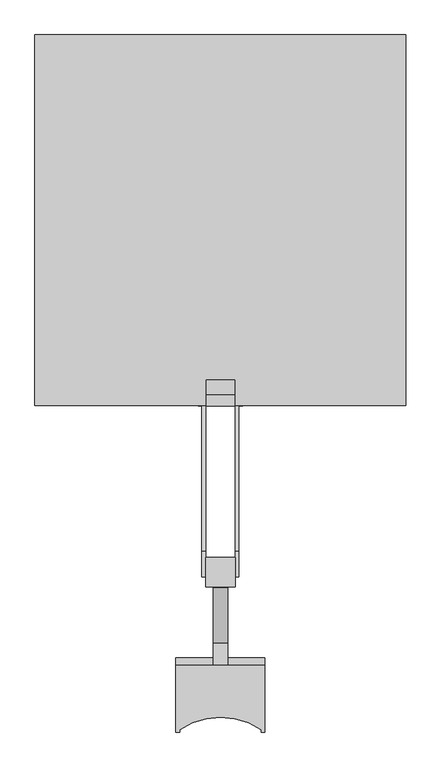
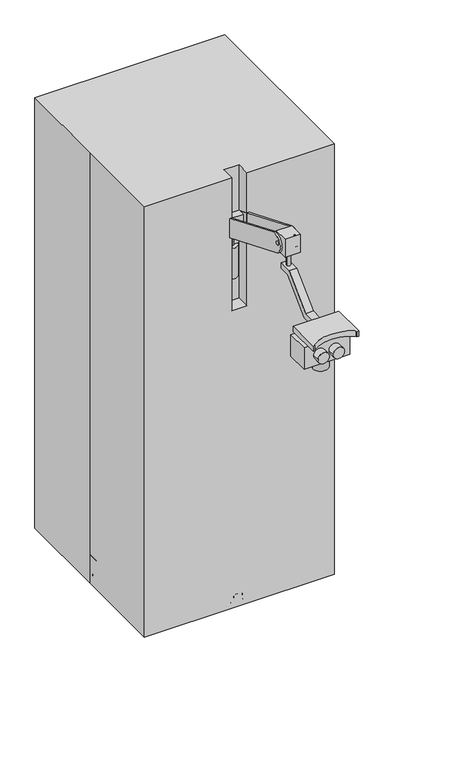
"""IFC4 building model written with IfcOpenShell, lengths in millimetres: proxy geometry, M8535 - Microscope, Operating, Portable : M8535 - Microscope, Operating, Portable."""

import ifcopenshell
import ifcopenshell.guid

model = None  # the IFC model being written
_history = None  # IfcOwnerHistory: only IFC2X3 demands one
_inside = {}  # id of a spatial element -> (the spatial element, [elements in it])
_under = {}  # id of a project, library or spatial element -> (it, [spatial elements below it])
_declared = {}  # id of a project -> (the project, [libraries it declares])
_typed = {}  # id of a type object -> (the type object, [elements of that type])
_made_of = {}  # id of a material, layer set ... -> (it, [elements and type objects made of it])


def new_model(schema):
    """Start an empty IFC model of exactly this schema.

    Asked for "IFC4X3", IfcOpenShell would pick the latest addendum, in which some entities
    have other attributes; the version numbers below select the first issue.
    IFC2X3 requires an IfcOwnerHistory on every rooted entity: one is made here for all.
    """
    global model, _history
    if schema == "IFC4X3":
        model = ifcopenshell.file(schema_version=(4, 3, 0, 0))
    else:
        model = ifcopenshell.file(schema=schema)
    _inside.clear()
    _under.clear()
    _declared.clear()
    _typed.clear()
    _made_of.clear()
    _history = None
    if model.schema == "IFC2X3":
        org = make("IfcOrganization", Name="unknown")
        user = make(
            "IfcPersonAndOrganization",
            ThePerson=make("IfcPerson", FamilyName="unknown"),
            TheOrganization=org,
        )
        app = make(
            "IfcApplication",
            ApplicationDeveloper=org,
            Version="unknown",
            ApplicationFullName="unknown",
            ApplicationIdentifier="unknown",
        )
        _history = make(
            "IfcOwnerHistory",
            OwningUser=user,
            OwningApplication=app,
            ChangeAction="ADDED",
            CreationDate=0,
        )
    return model


def make(cls, **values):
    """One entity of the class cls with the attributes given. An attribute that is None is left unset."""
    return model.create_entity(
        cls, **{name: value for name, value in values.items() if value is not None}
    )


def rooted(cls, **values):
    """An entity with a GlobalId (a new one), such as an element, a storey or a relation."""
    return make(cls, GlobalId=ifcopenshell.guid.new(), OwnerHistory=_history, **values)


def si_unit(unit_type, name, prefix=None):
    """IfcSIUnit, for example si_unit("LENGTHUNIT", "METRE", prefix="MILLI")."""
    return make("IfcSIUnit", UnitType=unit_type, Prefix=prefix, Name=name)


def assignment(units):
    """IfcUnitAssignment: the units of a project."""
    return None if units is None else make("IfcUnitAssignment", Units=units)


def point(xyz):
    """IfcCartesianPoint."""
    return None if xyz is None else make("IfcCartesianPoint", Coordinates=xyz)


def direction(xyz):
    """IfcDirection."""
    return None if xyz is None else make("IfcDirection", DirectionRatios=xyz)


def frame(location, z_axis=None, x_axis=None):
    """IfcAxis2Placement3D, a coordinate frame: its origin and axes. An axis left out is left unset."""
    return make(
        "IfcAxis2Placement3D",
        Location=point(location),
        Axis=direction(z_axis),
        RefDirection=direction(x_axis),
    )


def frame_2d(location, x_axis=None):
    """IfcAxis2Placement2D, a coordinate frame in the plane: its origin and x axis."""
    return make(
        "IfcAxis2Placement2D", Location=point(location), RefDirection=direction(x_axis)
    )


def origin():
    """The frame at (0, 0, 0) with its axes left unset."""
    return frame((0.0, 0.0, 0.0))


def origin_2d():
    """The frame at (0, 0) in the plane with its x axis left unset."""
    return frame_2d((0.0, 0.0))


def place(relative_to, where):
    """IfcLocalPlacement: puts the frame where relative to a parent placement (None: the world)."""
    return make(
        "IfcLocalPlacement", PlacementRelTo=relative_to, RelativePlacement=where
    )


def context(
    kind, dimensions, precision=None, world=None, true_north=None, identifier=None
):
    """IfcGeometricRepresentationContext, for example the 3D "Model" context."""
    return make(
        "IfcGeometricRepresentationContext",
        ContextIdentifier=identifier,
        ContextType=kind,
        CoordinateSpaceDimension=dimensions,
        Precision=precision,
        WorldCoordinateSystem=world,
        TrueNorth=true_north,
    )


def project(units=None, contexts=None):
    """IfcProject with its units and contexts."""
    return rooted(
        "IfcProject",
        Name="project",
        RepresentationContexts=contexts,
        UnitsInContext=assignment(units),
    )


def spatial(cls, under=None, at=None, **own):
    """A site, building, storey or space (cls), placed at a placement, below another one or the project."""
    s = rooted(cls, ObjectPlacement=at, **own)
    if under is not None:
        _under.setdefault(under.id(), (under, []))[1].append(s)
    return s


def polyline(points):
    """IfcPolyline through the points."""
    return make("IfcPolyline", Points=[point(p) for p in points])


def circle_curve(where, radius):
    """IfcCircle in the frame where."""
    return make("IfcCircle", Position=where, Radius=radius)


def ellipse_curve(where, semi_axis1, semi_axis2):
    """IfcEllipse in the frame where."""
    return make(
        "IfcEllipse", Position=where, SemiAxis1=semi_axis1, SemiAxis2=semi_axis2
    )


def trimmed(basis, trim1, trim2, sense, master):
    """IfcTrimmedCurve: the piece of a basis curve between two trims."""
    return make(
        "IfcTrimmedCurve",
        BasisCurve=basis,
        Trim1=trim1,
        Trim2=trim2,
        SenseAgreement=sense,
        MasterRepresentation=master,
    )


def segment(curve, same_sense, transition):
    """IfcCompositeCurveSegment."""
    return make(
        "IfcCompositeCurveSegment",
        Transition=transition,
        SameSense=same_sense,
        ParentCurve=curve,
    )


def composite_curve(segments, self_intersect=None):
    """IfcCompositeCurve: segments joined end to end."""
    return make("IfcCompositeCurve", Segments=segments, SelfIntersect=self_intersect)


def outline(outer, holes=None, kind="AREA"):
    """IfcArbitraryClosedProfileDef: a profile drawn as a closed curve; with holes, ...WithVoids."""
    if holes is None:
        return make("IfcArbitraryClosedProfileDef", ProfileType=kind, OuterCurve=outer)
    return make(
        "IfcArbitraryProfileDefWithVoids",
        ProfileType=kind,
        OuterCurve=outer,
        InnerCurves=holes,
    )


def extrude(swept, where, along, depth):
    """IfcExtrudedAreaSolid: the profile swept, set in the frame where, extruded along a direction by depth."""
    return make(
        "IfcExtrudedAreaSolid",
        SweptArea=swept,
        Position=where,
        ExtrudedDirection=direction(along),
        Depth=depth,
    )


def faces_of(points, faces, orient=None, outer=None):
    """IfcFace entities. A face is a list of loops; a loop is a list of indices into points, from 0.

    orient and outer hold one flag for each loop. By default every Orientation is true, the
    first loop of a face is its IfcFaceOuterBound and the others are IfcFaceBound.
    """
    made = []
    for i, loops in enumerate(faces):
        bounds = []
        for j, loop in enumerate(loops):
            is_outer = j == 0 if outer is None else outer[i][j]
            bounds.append(
                make(
                    "IfcFaceOuterBound" if is_outer else "IfcFaceBound",
                    Bound=make("IfcPolyLoop", Polygon=[points[k] for k in loop]),
                    Orientation=True if orient is None else orient[i][j],
                )
            )
        made.append(make("IfcFace", Bounds=bounds))
    return made


def faceted_brep(points, faces, orient=None, outer=None, voids=None):
    """IfcFacetedBrep: a solid bounded by flat faces; with voids (closed shells), ...WithVoids."""
    shared = [point(p) for p in points]
    hull = make("IfcClosedShell", CfsFaces=faces_of(shared, faces, orient, outer))
    if voids is None:
        return make("IfcFacetedBrep", Outer=hull)
    return make(
        "IfcFacetedBrepWithVoids",
        Outer=hull,
        Voids=[
            make(cls, CfsFaces=faces_of(shared, fs, o, b)) for cls, fs, o, b in voids
        ],
    )


def shape(context_of_items, identifier, shape_type, items):
    """IfcShapeRepresentation: the items that make up one representation, for example the "Body"."""
    return make(
        "IfcShapeRepresentation",
        ContextOfItems=context_of_items,
        RepresentationIdentifier=identifier,
        RepresentationType=shape_type,
        Items=items,
    )


def source(mapping_origin, context_of_items, identifier, shape_type, items):
    """IfcRepresentationMap: a shape defined once, which mapped items show again and again."""
    return make(
        "IfcRepresentationMap",
        MappingOrigin=mapping_origin,
        MappedRepresentation=shape(context_of_items, identifier, shape_type, items),
    )


def transform(
    local_origin,
    x_axis=None,
    y_axis=None,
    z_axis=None,
    scale=None,
    scale2=None,
    scale3=None,
    uniform=True,
):
    """IfcCartesianTransformationOperator3D, or its non-uniform kind. x_axis, y_axis, z_axis: its Axis1, 2, 3."""
    if uniform:
        return make(
            "IfcCartesianTransformationOperator3D",
            Axis1=direction(x_axis),
            Axis2=direction(y_axis),
            LocalOrigin=point(local_origin),
            Scale=scale,
            Axis3=direction(z_axis),
        )
    return make(
        "IfcCartesianTransformationOperator3DnonUniform",
        Axis1=direction(x_axis),
        Axis2=direction(y_axis),
        LocalOrigin=point(local_origin),
        Scale=scale,
        Axis3=direction(z_axis),
        Scale2=scale2,
        Scale3=scale3,
    )


def mapped(mapping_source, mapping_target):
    """IfcMappedItem: shows the shape of a source again, moved by a transform."""
    return make(
        "IfcMappedItem", MappingSource=mapping_source, MappingTarget=mapping_target
    )


def made_of(thing, what):
    """Note that an element or type object is made of a material, layer set ...; save() writes the relation."""
    if what is not None:
        _made_of.setdefault(what.id(), (what, []))[1].append(thing)
    return thing


def element(
    cls,
    number,
    at=None,
    inside=None,
    cuts=None,
    type_object=None,
    material=None,
    context=None,
    identifier="Body",
    shape_type=None,
    held_by="IfcProductDefinitionShape",
    body=None,
    shapes=None,
    **own,
):
    """One element of the class cls, such as IfcWall. Its Tag is "e" and its number.

    at: its placement. inside: the storey or other place that contains it. cuts: it is an
    opening in that element (IfcRelVoidsElement). A single representation is given by context,
    identifier, shape_type and body (its items); several are given by shapes. held_by: the class
    of the entity that holds the representations. save() writes the other relations.
    """
    e = rooted(cls, Tag="e%d" % number, ObjectPlacement=at, **own)
    if body is not None:
        shapes = [shape(context, identifier, shape_type, body)]
    if shapes is not None:
        e.Representation = make(held_by, Representations=shapes)
    if inside is not None:
        _inside.setdefault(inside.id(), (inside, []))[1].append(e)
    if cuts is not None:
        rooted(
            "IfcRelVoidsElement", RelatingBuildingElement=cuts, RelatedOpeningElement=e
        )
    if type_object is not None:
        _typed.setdefault(type_object.id(), (type_object, []))[1].append(e)
    return made_of(e, material)


def aggregate(whole, parts):
    """IfcRelAggregates: a whole, such as a stair, and the parts it consists of."""
    return rooted("IfcRelAggregates", RelatingObject=whole, RelatedObjects=parts)


def save(model, path):
    """Write the relations noted so far, then the file.

    IfcRelAggregates (storeys below a building ...), IfcRelContainedInSpatialStructure (elements
    in a storey), IfcRelDefinesByType, IfcRelAssociatesMaterial and IfcRelDeclares: one each for
    every whole, place, type object, material and project.
    """
    for whole, parts in _under.values():
        aggregate(whole, parts)
    for where, things in _inside.values():
        rooted(
            "IfcRelContainedInSpatialStructure",
            RelatedElements=things,
            RelatingStructure=where,
        )
    for kind, things in _typed.values():
        rooted("IfcRelDefinesByType", RelatedObjects=things, RelatingType=kind)
    for what, things in _made_of.values():
        rooted("IfcRelAssociatesMaterial", RelatedObjects=things, RelatingMaterial=what)
    for by, libraries in _declared.values():
        rooted("IfcRelDeclares", RelatingContext=by, RelatedDefinitions=libraries)
    model.write(path)


def plane_surface(at):
    """IfcPlane: the flat surface through the origin of the frame at, square to its z axis."""
    return make("IfcPlane", Position=at)


def cylinder_surface(at, radius):
    """IfcCylindricalSurface: all points at the distance radius from the z axis of the frame at."""
    return make("IfcCylindricalSurface", Position=at, Radius=radius)


def revolved_surface(curve, axis_point, axis_direction):
    """IfcSurfaceOfRevolution: the curve turned about the line through axis_point along axis_direction."""
    return make(
        "IfcSurfaceOfRevolution",
        SweptCurve=make("IfcArbitraryOpenProfileDef", ProfileType="CURVE", Curve=curve),
        AxisPosition=make("IfcAxis1Placement", Location=point(axis_point), Axis=direction(axis_direction)),
    )


def extruded_surface(curve, direction_of_extrusion, depth):
    """IfcSurfaceOfLinearExtrusion: the curve pushed along a direction by depth."""
    return make(
        "IfcSurfaceOfLinearExtrusion",
        SweptCurve=make("IfcArbitraryOpenProfileDef", ProfileType="CURVE", Curve=curve),
        ExtrudedDirection=direction(direction_of_extrusion),
        Depth=depth,
    )


def advanced_brep(points, edges, surfaces, faces):
    """IfcAdvancedBrep: a solid bounded by faces that lie on surfaces and meet in shared edges.

    An edge is (start, end): straight between two places in points (the first is 0);
    or (start, end, curve); or (start, end, curve, False) where it runs against its curve.
    A face is (place in surfaces, loops), or (place, loops, False) where it looks against
    its surface's normal. A loop lists edges by number (the first is 1), with a minus sign
    where the edge is run from its end to its start. The first loop is the outer one.
    """
    corners = [point(p) for p in points]
    vertices = [make("IfcVertexPoint", VertexGeometry=c) for c in corners]
    made = []
    for start, end, *more in edges:
        made.append(
            make(
                "IfcEdgeCurve",
                EdgeStart=vertices[start],
                EdgeEnd=vertices[end],
                EdgeGeometry=more[0] if more else make("IfcPolyline", Points=[corners[start], corners[end]]),
                SameSense=more[1] if len(more) > 1 else True,
            )
        )
    hull = []
    for where, loops, *sense in faces:
        bounds = []
        for j, loop in enumerate(loops):
            ring = [make("IfcOrientedEdge", EdgeElement=made[abs(k) - 1], Orientation=k > 0) for k in loop]
            bounds.append(
                make(
                    "IfcFaceOuterBound" if j == 0 else "IfcFaceBound",
                    Bound=make("IfcEdgeLoop", EdgeList=ring),
                    Orientation=True,
                )
            )
        hull.append(make("IfcAdvancedFace", Bounds=bounds, FaceSurface=surfaces[where], SameSense=sense[0] if sense else True))
    return make("IfcAdvancedBrep", Outer=make("IfcClosedShell", CfsFaces=hull))


def specialty_equipment_8152f2bc(model_context):
    return source(origin(), model_context, "Body", "SolidModel", [
        advanced_brep(
        [(31.75, -590.6759875, 1426.2297914), (31.75, -309.077506, 1309.5878812), (31.75, -284.777108, 1368.2542315), (31.75, -566.3755895, 1484.8961417), (31.75, -284.6907592, 1326.9793218), (31.75, -279.8306796, 1338.7125919), (31.75, -595.6224159, 1455.771431), (31.75, -590.7623363, 1467.5047011), (-31.75, -590.6759875, 1426.2297914), (-31.75, -566.3755895, 1484.8961417), (-31.75, -284.777108, 1368.2542315), (-31.75, -309.077506, 1309.5878812), (-31.75, -284.6907592, 1326.9793218), (-31.75, -279.8306796, 1338.7125919), (-31.75, -595.6224159, 1455.771431), (-31.75, -590.7623363, 1467.5047011), (25.4, -590.6759875, 1426.2297914), (25.4, -309.077506, 1309.5878812), (-25.4, -309.077506, 1309.5878812), (-25.4, -590.6759875, 1426.2297914), (25.4, -272.6761469, 1318.4285276), (-25.4, -272.6761469, 1318.4285276), (-25.4, -284.777108, 1368.2542315), (-25.4, -272.6761469, 1359.4135851), (25.4, -272.6761469, 1359.4135851), (25.4, -284.777108, 1368.2542315), (25.4, -566.3755895, 1484.8961417), (-25.4, -566.3755895, 1484.8961417), (25.4, -602.5772402, 1476.2895237), (-25.4, -602.5772402, 1476.2895237), (-25.4, -602.5772402, 1434.8364095), (25.4, -602.5772402, 1434.8364095), (25.4, -284.6907592, 1326.9793218), (25.4, -279.8306796, 1338.7125919), (-25.4, -279.8306796, 1338.7125919), (-25.4, -284.6907592, 1326.9793218), (25.4, -595.6224159, 1455.771431), (25.4, -590.7623363, 1467.5047011), (-25.4, -590.7623363, 1467.5047011), (-25.4, -595.6224159, 1455.771431)],
        [
            (0, 1),
            (1, 2, circle_curve(frame((31.75, -296.927307, 1338.9210564), z_axis=(1.0, 0.0, 0.0), x_axis=(0.0, 0.3826834323650877, 0.9238795325112876)), 31.75)),
            (2, 3),
            (3, 0, circle_curve(frame((31.75, -578.5257885, 1455.5629666), z_axis=(1.0, 0.0, 0.0), x_axis=(0.0, 0.3826834323650936, 0.9238795325112853)), 31.75)),
            (4, 5, circle_curve(frame((31.75, -282.2607194, 1332.8459569), z_axis=(-1.0, 0.0, 0.0), x_axis=(0.0, 0.3826834323650877, 0.9238795325112876)), 6.35)),
            (5, 4, circle_curve(frame((31.75, -282.2607194, 1332.8459569), z_axis=(-1.0, 0.0, 0.0), x_axis=(0.0, 0.3826834323650877, 0.9238795325112876)), 6.35)),
            (6, 7, circle_curve(frame((31.75, -593.1923761, 1461.638066), z_axis=(-1.0, 0.0, 0.0), x_axis=(0.0, 0.3826834323650936, 0.9238795325112853)), 6.35)),
            (7, 6, circle_curve(frame((31.75, -593.1923761, 1461.638066), z_axis=(-1.0, 0.0, 0.0), x_axis=(0.0, 0.3826834323650936, 0.9238795325112853)), 6.35)),
            (8, 9, circle_curve(frame((-31.75, -578.5257885, 1455.5629666), z_axis=(-1.0, 0.0, 0.0), x_axis=(0.0, 0.3826834323650936, 0.9238795325112853)), 31.75)),
            (9, 10),
            (10, 11, circle_curve(frame((-31.75, -296.927307, 1338.9210564), z_axis=(-1.0, 0.0, 0.0), x_axis=(0.0, 0.3826834323650877, 0.9238795325112876)), 31.75)),
            (11, 8),
            (12, 13, circle_curve(frame((-31.75, -282.2607194, 1332.8459569), z_axis=(1.0, 0.0, 0.0), x_axis=(0.0, 0.3826834323650877, 0.9238795325112876)), 6.35)),
            (13, 12, circle_curve(frame((-31.75, -282.2607194, 1332.8459569), z_axis=(1.0, 0.0, 0.0), x_axis=(0.0, 0.3826834323650877, 0.9238795325112876)), 6.35)),
            (14, 15, circle_curve(frame((-31.75, -593.1923761, 1461.638066), z_axis=(1.0, 0.0, 0.0), x_axis=(0.0, 0.3826834323650936, 0.9238795325112853)), 6.35)),
            (15, 14, circle_curve(frame((-31.75, -593.1923761, 1461.638066), z_axis=(1.0, 0.0, 0.0), x_axis=(0.0, 0.3826834323650936, 0.9238795325112853)), 6.35)),
            (0, 16),
            (16, 17),
            (17, 1),
            (11, 18),
            (18, 19),
            (19, 8),
            (17, 20, circle_curve(frame((25.4, -296.927307, 1338.9210564), z_axis=(1.0, 0.0, 0.0), x_axis=(0.0, 0.3826834323650877, 0.9238795325112876)), 31.75)),
            (20, 21),
            (21, 18, circle_curve(frame((-25.4, -296.927307, 1338.9210564), z_axis=(-1.0, 0.0, 0.0), x_axis=(0.0, 0.3826834323650877, 0.9238795325112876)), 31.75)),
            (10, 22),
            (22, 23, circle_curve(frame((-25.4, -296.927307, 1338.9210564), z_axis=(-1.0, 0.0, 0.0), x_axis=(0.0, 0.3826834323650877, 0.9238795325112876)), 31.75)),
            (23, 24),
            (24, 25, circle_curve(frame((25.4, -296.927307, 1338.9210564), z_axis=(1.0, 0.0, 0.0), x_axis=(0.0, 0.3826834323650877, 0.9238795325112876)), 31.75)),
            (25, 2),
            (25, 26),
            (26, 3),
            (9, 27),
            (27, 22),
            (26, 28, circle_curve(frame((25.4, -578.5257885, 1455.5629666), z_axis=(1.0, 0.0, 0.0), x_axis=(0.0, 0.3826834323650936, 0.9238795325112853)), 31.75)),
            (28, 29),
            (29, 27, circle_curve(frame((-25.4, -578.5257885, 1455.5629666), z_axis=(-1.0, 0.0, 0.0), x_axis=(0.0, 0.3826834323650936, 0.9238795325112853)), 31.75)),
            (19, 30, circle_curve(frame((-25.4, -578.5257885, 1455.5629666), z_axis=(-1.0, 0.0, 0.0), x_axis=(0.0, 0.3826834323650936, 0.9238795325112853)), 31.75)),
            (30, 31),
            (31, 16, circle_curve(frame((25.4, -578.5257885, 1455.5629666), z_axis=(1.0, 0.0, 0.0), x_axis=(0.0, 0.3826834323650936, 0.9238795325112853)), 31.75)),
            (4, 32),
            (32, 33, circle_curve(frame((25.4, -282.2607194, 1332.8459569), z_axis=(-1.0, 0.0, 0.0), x_axis=(0.0, 0.3826834323650877, 0.9238795325112876)), 6.35)),
            (33, 5),
            (13, 34),
            (34, 35, circle_curve(frame((-25.4, -282.2607194, 1332.8459569), z_axis=(1.0, 0.0, 0.0), x_axis=(0.0, 0.3826834323650877, 0.9238795325112876)), 6.35)),
            (35, 12),
            (33, 32, circle_curve(frame((25.4, -282.2607194, 1332.8459569), z_axis=(-1.0, 0.0, 0.0), x_axis=(0.0, 0.3826834323650877, 0.9238795325112876)), 6.35)),
            (35, 34, circle_curve(frame((-25.4, -282.2607194, 1332.8459569), z_axis=(1.0, 0.0, 0.0), x_axis=(0.0, 0.3826834323650877, 0.9238795325112876)), 6.35)),
            (6, 36),
            (36, 37, circle_curve(frame((25.4, -593.1923761, 1461.638066), z_axis=(-1.0, 0.0, 0.0), x_axis=(0.0, 0.3826834323650936, 0.9238795325112853)), 6.35)),
            (37, 7),
            (15, 38),
            (38, 39, circle_curve(frame((-25.4, -593.1923761, 1461.638066), z_axis=(1.0, 0.0, 0.0), x_axis=(0.0, 0.3826834323650936, 0.9238795325112853)), 6.35)),
            (39, 14),
            (37, 36, circle_curve(frame((25.4, -593.1923761, 1461.638066), z_axis=(-1.0, 0.0, 0.0), x_axis=(0.0, 0.3826834323650936, 0.9238795325112853)), 6.35)),
            (39, 38, circle_curve(frame((-25.4, -593.1923761, 1461.638066), z_axis=(1.0, 0.0, 0.0), x_axis=(0.0, 0.3826834323650936, 0.9238795325112853)), 6.35)),
            (21, 23),
            (29, 30),
            (28, 31),
            (24, 20),
        ],
        [
            plane_surface(frame((31.75, -309.077506, 1309.5878812), z_axis=(1.0000000000000002, 0.0, 0.0), x_axis=(0.0, 0.9238795325112863, -0.382683432365091))),
            plane_surface(frame((-31.75, -309.077506, 1309.5878812), z_axis=(-1.0000000000000002, 0.0, 0.0), x_axis=(0.0, -0.9238795325112863, 0.382683432365091))),
            plane_surface(frame((31.75, -590.6759875, 1426.2297914), z_axis=(0.0, -0.382683432365091, -0.9238795325112863), x_axis=(-1.0, 0.0, 0.0))),
            cylinder_surface(frame((-31.75, -296.927307, 1338.9210564), z_axis=(1.0, 0.0, 0.0), x_axis=(0.0, 0.3826834323650877, 0.9238795325112876)), 31.75),
            plane_surface(frame((31.75, -284.777108, 1368.2542315), z_axis=(0.0, 0.38268343236509117, 0.9238795325112863), x_axis=(-1.0, 0.0, 0.0))),
            cylinder_surface(frame((-31.75, -578.5257885, 1455.5629666), z_axis=(1.0000000000000002, 0.0, 0.0), x_axis=(0.0, 0.3826834323650936, 0.9238795325112853)), 31.75),
            revolved_surface(polyline([(25.4, -279.8306796044817, 1338.7125919314467), (31.75, -279.8306796044817, 1338.7125919314467)]), (0.0, -282.2607194, 1332.8459569), (-1.0, 0.0, 0.0)),
            revolved_surface(polyline([(-31.75, -279.8306796044817, 1338.7125919314467), (-25.4, -279.8306796044817, 1338.7125919314467)]), (0.0, -282.2607194, 1332.8459569), (-1.0, 0.0, 0.0)),
            revolved_surface(polyline([(25.400000000000013, -590.7623363044817, 1467.5047010314465), (31.750000000000014, -590.7623363044817, 1467.5047010314465)]), (0.0, -593.1923761, 1461.638066), (-1.0000000000000002, 0.0, 0.0)),
            revolved_surface(polyline([(-31.750000000000014, -590.7623363044817, 1467.5047010314465), (-25.400000000000013, -590.7623363044817, 1467.5047010314465)]), (0.0, -593.1923761, 1461.638066), (-1.0000000000000002, 0.0, 0.0)),
            plane_surface(frame((-25.4, -272.6761469, 1742.3404738), z_axis=(1.0, 0.0, 0.0), x_axis=(0.0, 0.0, -1.0))),
            plane_surface(frame((-25.4, -602.5772402, 1742.3404738), z_axis=(0.0, 1.0, 0.0), x_axis=(0.0, 0.0, -1.0))),
            plane_surface(frame((25.4, -602.5772402, 1742.3404738), z_axis=(-1.0, 0.0, 0.0), x_axis=(0.0, 0.0, -1.0))),
            plane_surface(frame((25.4, -272.6761469, 1742.3404738), z_axis=(0.0, -1.0, 0.0), x_axis=(0.0, 0.0, -1.0))),
        ],
        [
            (0, [[1, 2, 3, 4], [5, 6], [7, 8]]),
            (1, [[9, 10, 11, 12], [13, 14], [15, 16]]),
            (2, [[-1, 17, 18, 19]]),
            (2, [[-12, 20, 21, 22]]),
            (3, [[-2, -19, 23, 24, 25, -20, -11, 26, 27, 28, 29, 30]]),
            (4, [[-3, -30, 31, 32]]),
            (4, [[-10, 33, 34, -26]]),
            (5, [[-4, -32, 35, 36, 37, -33, -9, -22, 38, 39, 40, -17]]),
            (6, [[-5, 41, 42, 43]]),
            (7, [[-14, 44, 45, 46]]),
            (6, [[-6, -43, 47, -41]]),
            (7, [[-13, -46, 48, -44]]),
            (8, [[-7, 49, 50, 51]]),
            (9, [[-16, 52, 53, 54]]),
            (8, [[-8, -51, 55, -49]]),
            (9, [[-15, -54, 56, -52]]),
            (10, [[57, -27, -34, -37, 58, -38, -21, -25], [-45, -48], [-53, -56]]),
            (11, [[-58, -36, 59, -39]]),
            (12, [[-59, -35, -31, -29, 60, -23, -18, -40], [-42, -47], [-50, -55]]),
            (13, [[-57, -24, -60, -28]]),
        ],
    ),
        extrude(outline(composite_curve([segment(trimmed(circle_curve(frame_2d((0.0, -276.3595017)), 9.525), [point((-9.525, -276.3595017))], [point((9.525, -276.3595017))], False, "CARTESIAN"), True, "CONTINUOUS"), segment(trimmed(circle_curve(frame_2d((0.0, -276.3595017)), 9.525), [point((9.525, -276.3595017))], [point((-9.525, -276.3595017))], False, "CARTESIAN"), True, "CONTINUOUS")], self_intersect=False)), frame((0.0, 0.0, 38.9774203), z_axis=(0.0, 0.0, 1.0), x_axis=(1.0, 0.0, 0.0)), (0.0, 0.0, 1.0), 49.9225797),
        faceted_brep([(-317.5, 317.5, 1524.0), (-317.5, 0.0, 1524.0), (-317.5, -317.5, 1524.0), (-25.4, -317.5, 1524.0), (-25.4, -272.6761469, 1524.0), (25.4, -272.6761469, 1524.0), (25.4, -317.5, 1524.0), (317.5, -317.5, 1524.0), (317.5, 317.5, 1524.0), (-317.5, 317.5, 0.0), (317.5, 317.5, 0.0), (317.5, -317.5, 0.0), (-317.5, -317.5, 0.0), (-317.5, 0.0, 0.0), (25.4, -317.5, 1053.5091843), (-25.4, -317.5, 1053.5091843), (25.4, -272.6761469, 1053.5091843), (-25.4, -272.6761469, 1053.5091843)], [[[0, 1, 2, 3, 4, 5, 6, 7, 8]], [[9, 10, 11, 12, 13]], [[1, 0, 9, 13]], [[2, 1, 13, 12]], [[12, 11, 7, 6, 14, 15, 3, 2]], [[8, 7, 11, 10]], [[0, 8, 10, 9]], [[16, 17, 15, 14]], [[15, 17, 4, 3]], [[16, 14, 6, 5]], [[17, 16, 5, 4]]]),
        extrude(outline(polyline([(-253.6261469, 1142.6261469), (-253.6261469, 1250.3892204), (38.1, 958.6630735), (38.1, 927.1), (-38.1, 927.1), (-253.6261469, 1142.6261469)])), frame((-25.4, 0.0, 0.0), z_axis=(1.0, 0.0, 0.0), x_axis=(0.0, 1.0, 0.0)), (0.0, 0.0, 1.0), 50.8),
        extrude(outline(composite_curve([segment(trimmed(circle_curve(frame_2d((0.0, -787.3125604)), 25.4), [point((-25.4, -787.3125604))], [point((25.4, -787.3125604))], False, "CARTESIAN"), True, "CONTINUOUS"), segment(trimmed(circle_curve(frame_2d((0.0, -787.3125604)), 25.4), [point((25.4, -787.3125604))], [point((-25.4, -787.3125604))], False, "CARTESIAN"), True, "CONTINUOUS")], self_intersect=False)), frame((0.0, 0.0, 1132.7881292), z_axis=(0.0, 0.0, 1.0), x_axis=(1.0, 0.0, 0.0)), (0.0, 0.0, 1.0), 38.1),
        extrude(outline(composite_curve([segment(trimmed(circle_curve(frame_2d((1208.9881292, -25.4)), 19.05), [point((1208.9881292, -44.45))], [point((1208.9881292, -6.35))], False, "CARTESIAN"), True, "CONTINUOUS"), segment(trimmed(circle_curve(frame_2d((1208.9881292, -25.4)), 19.05), [point((1208.9881292, -6.35))], [point((1208.9881292, -44.45))], False, "CARTESIAN"), True, "CONTINUOUS")], self_intersect=False)), frame((0.0, -850.8125604, 0.0), z_axis=(0.0, 1.0, 0.0), x_axis=(0.0, 0.0, 1.0)), (0.0, 0.0, 1.0), 25.4),
        extrude(outline(composite_curve([segment(trimmed(circle_curve(frame_2d((1208.9881292, 25.4)), 19.05), [point((1208.9881292, 6.35))], [point((1208.9881292, 44.45))], False, "CARTESIAN"), True, "CONTINUOUS"), segment(trimmed(circle_curve(frame_2d((1208.9881292, 25.4)), 19.05), [point((1208.9881292, 44.45))], [point((1208.9881292, 6.35))], False, "CARTESIAN"), True, "CONTINUOUS")], self_intersect=False)), frame((0.0, -850.8125604, 0.0), z_axis=(0.0, 1.0, 0.0), x_axis=(0.0, 0.0, 1.0)), (0.0, 0.0, 1.0), 25.4),
        extrude(outline(polyline([(76.2, -749.2125604), (76.2, -825.4125604), (-76.2, -825.4125604), (-76.2, -749.2125604), (76.2, -749.2125604)])), frame((0.0, 0.0, 1170.8881292), z_axis=(0.0, 0.0, 1.0), x_axis=(1.0, 0.0, 0.0)), (0.0, 0.0, 1.0), 76.2),
        extrude(outline(composite_curve([segment(trimmed(circle_curve(frame_2d((0.0, -787.3125604)), 3.175), [point((0.0, -784.1375604))], [point((0.0, -790.4875604))], False, "CARTESIAN"), True, "CONTINUOUS"), segment(trimmed(circle_curve(frame_2d((0.0, -787.3125604)), 3.175), [point((0.0, -790.4875604))], [point((0.0, -784.1375604))], False, "CARTESIAN"), True, "CONTINUOUS")], self_intersect=False)), frame((0.0, 0.0, 1247.0881292), z_axis=(0.0, 0.0, 1.0), x_axis=(1.0, 0.0, 0.0)), (0.0, 0.0, 1.0), 19.05),
        extrude(outline(composite_curve([segment(polyline([(-76.2, -761.9125604), (76.2, -761.9125604), (76.2, -877.0164384), (69.85, -877.0164384), (69.85, -872.5173882)]), True, "CONTINUOUS"), segment(trimmed(circle_curve(frame_2d((0.0, -974.8456023)), 123.8954636), [point((69.85, -872.5173882))], [point((-69.85, -872.5173882))], True, "CARTESIAN"), True, "CONTINUOUS"), segment(polyline([(-69.85, -872.5173882), (-69.85, -877.0164384), (-76.2, -877.0164384), (-76.2, -761.9125604)]), True, "CONTINUOUS")], self_intersect=False)), frame((0.0, 0.0, 1266.1381292), z_axis=(0.0, 0.0, 1.0), x_axis=(1.0, 0.0, 0.0)), (0.0, 0.0, 1.0), 19.05),
        extrude(outline(polyline([(-629.5180086, 1379.482681), (-583.5272402, 1379.482681), (-583.5272402, 1360.432681), (-621.6272402, 1360.432681), (-715.921792, 1266.1381292), (-761.9125604, 1266.1381292), (-761.9125604, 1285.1881292), (-723.8125604, 1285.1881292), (-629.5180086, 1379.482681)])), frame((-12.7, 0.0, 0.0), z_axis=(1.0, 0.0, 0.0), x_axis=(0.0, 1.0, 0.0)), (0.0, 0.0, 1.0), 25.4),
        extrude(outline(composite_curve([segment(trimmed(circle_curve(frame_2d((0.0, -602.5772402)), 6.35), [point((-6.35, -602.5772402))], [point((6.35, -602.5772402))], False, "CARTESIAN"), True, "CONTINUOUS"), segment(trimmed(circle_curve(frame_2d((0.0, -602.5772402)), 6.35), [point((6.35, -602.5772402))], [point((-6.35, -602.5772402))], False, "CARTESIAN"), True, "CONTINUOUS")], self_intersect=False)), frame((0.0, 0.0, 1379.482681), z_axis=(0.0, 0.0, 1.0), x_axis=(1.0, 0.0, 0.0)), (0.0, 0.0, 1.0), 50.8),
        extrude(outline(polyline([(25.4, -577.1772402), (25.4, -627.9772402), (-25.4, -627.9772402), (-25.4, -577.1772402), (25.4, -577.1772402)])), frame((0.0, 0.0, 1430.282681), z_axis=(0.0, 0.0, 1.0), x_axis=(1.0, 0.0, 0.0)), (0.0, 0.0, 1.0), 63.5),
        extrude(outline(polyline([(25.4, -247.2761469), (25.4, -298.0761469), (-25.4, -298.0761469), (-25.4, -247.2761469), (25.4, -247.2761469)])), frame((0.0, 0.0, 1301.1892204), z_axis=(0.0, 0.0, 1.0), x_axis=(1.0, 0.0, 0.0)), (0.0, 0.0, 1.0), 63.5),
        extrude(outline(composite_curve([segment(trimmed(circle_curve(frame_2d((0.0, -272.6761469)), 6.35), [point((0.0, -266.3261469))], [point((0.0, -279.0261469))], False, "CARTESIAN"), True, "CONTINUOUS"), segment(trimmed(circle_curve(frame_2d((0.0, -272.6761469)), 6.35), [point((0.0, -279.0261469))], [point((0.0, -266.3261469))], False, "CARTESIAN"), True, "CONTINUOUS")], self_intersect=False)), frame((0.0, 0.0, 1250.3892204), z_axis=(0.0, 0.0, 1.0), x_axis=(1.0, 0.0, 0.0)), (0.0, 0.0, 1.0), 50.8),
        advanced_brep(
        [(-25.4, -253.6261469, 1250.3892204), (25.4, -253.6261469, 1250.3892204), (-25.4, -253.6261469, 1142.6261469), (25.4, -253.6261469, 1142.6261469)],
        [
            (0, 1, ellipse_curve(frame((0.0, -253.6261469, 1250.3892204), z_axis=(0.0, 0.0, 1.0), x_axis=(0.0, 1.0, 0.0)), 38.1, 25.4)),
            (1, 0),
            (2, 3),
            (3, 2, ellipse_curve(frame((0.0, -253.6261469, 1142.6261469), z_axis=(0.0, 0.0, -1.0), x_axis=(1.0, 0.0, 0.0)), 25.4, 38.1)),
            (1, 3),
            (2, 0),
        ],
        [
            plane_surface(frame((25.4, -253.6261469, 1250.3892204), z_axis=(0.0, 0.0, 1.0), x_axis=(0.0, 1.0, 0.0))),
            plane_surface(frame((25.4, -253.6261469, 1142.6261469), z_axis=(0.0, 0.0, -1.0), x_axis=(0.0, -1.0, 0.0))),
            plane_surface(frame((25.4, -253.6261469, 1250.3892204), z_axis=(0.0, 1.0, 0.0), x_axis=(0.0, 0.0, -1.0))),
            extruded_surface(trimmed(ellipse_curve(frame((0.0, -253.6261469, 1034.8630735), z_axis=(0.0, 0.0, 1.0), x_axis=(1.0, 0.0, 0.0)), 25.4, 38.1), [point((-25.4, -253.6261469, 1034.8630735))], [point((25.4, -253.6261469, 1034.8630735))], True, "CARTESIAN"), (0.0, 0.0, 107.76307340000017), 107.76307340000017),
        ],
        [
            (0, [[1, 2]]),
            (1, [[3, 4]]),
            (2, [[-2, 5, -3, 6]]),
            (3, [[-1, -6, -4, -5]]),
        ],
    ),
        extrude(outline(polyline([(76.2, 76.2), (76.2, -76.2), (-76.2, -76.2), (-76.2, 76.2), (76.2, 76.2)])), frame((0.0, 0.0, 914.4), z_axis=(0.0, 0.0, 1.0), x_axis=(1.0, 0.0, 0.0)), (0.0, 0.0, 1.0), 12.7),
        extrude(outline(composite_curve([segment(trimmed(circle_curve(origin_2d(), 38.1), [point((-38.1, 0.0))], [point((38.1, 0.0))], False, "CARTESIAN"), True, "CONTINUOUS"), segment(trimmed(circle_curve(origin_2d(), 38.1), [point((38.1, 0.0))], [point((-38.1, 0.0))], False, "CARTESIAN"), True, "CONTINUOUS")], self_intersect=False)), frame((0.0, 0.0, 203.2), z_axis=(0.0, 0.0, 1.0), x_axis=(1.0, 0.0, 0.0)), (0.0, 0.0, 1.0), 711.2),
        extrude(outline(composite_curve([segment(trimmed(circle_curve(origin_2d(), 53.8815367), [point((-53.8815367, 0.0))], [point((53.8815367, 0.0))], False, "CARTESIAN"), True, "CONTINUOUS"), segment(trimmed(circle_curve(origin_2d(), 53.8815367), [point((53.8815367, 0.0))], [point((-53.8815367, 0.0))], False, "CARTESIAN"), True, "CONTINUOUS")], self_intersect=False)), frame((0.0, 0.0, 101.6), z_axis=(0.0, 0.0, 1.0), x_axis=(1.0, 0.0, 0.0)), (0.0, 0.0, 1.0), 101.6),
        extrude(outline(composite_curve([segment(trimmed(circle_curve(frame_2d((276.3595017, 0.0)), 9.525), [point((276.3595017, 9.525))], [point((276.3595017, -9.525))], False, "CARTESIAN"), True, "CONTINUOUS"), segment(trimmed(circle_curve(frame_2d((276.3595017, 0.0)), 9.525), [point((276.3595017, -9.525))], [point((276.3595017, 9.525))], False, "CARTESIAN"), True, "CONTINUOUS")], self_intersect=False)), frame((0.0, 0.0, 38.9774203), z_axis=(0.0, 0.0, 1.0), x_axis=(1.0, 0.0, 0.0)), (0.0, 0.0, 1.0), 49.9225797),
        extrude(outline(composite_curve([segment(trimmed(circle_curve(frame_2d((38.1, 279.4)), 38.1), [point((38.1, 317.5))], [point((38.1, 241.3))], False, "CARTESIAN"), True, "CONTINUOUS"), segment(trimmed(circle_curve(frame_2d((38.1, 279.4)), 38.1), [point((38.1, 241.3))], [point((38.1, 317.5))], False, "CARTESIAN"), True, "CONTINUOUS")], self_intersect=False)), frame((0.0, 9.525, 0.0), z_axis=(0.0, 1.0, 0.0), x_axis=(0.0, 0.0, 1.0)), (0.0, 0.0, 1.0), 9.525),
        extrude(outline(composite_curve([segment(trimmed(circle_curve(frame_2d((38.1, 279.4623599)), 19.05), [point((38.1, 298.5123599))], [point((38.1, 260.4123599))], False, "CARTESIAN"), True, "CONTINUOUS"), segment(trimmed(circle_curve(frame_2d((38.1, 279.4623599)), 19.05), [point((38.1, 260.4123599))], [point((38.1, 298.5123599))], False, "CARTESIAN"), True, "CONTINUOUS")], self_intersect=False)), frame((0.0, -9.525, 0.0), z_axis=(0.0, 1.0, 0.0), x_axis=(0.0, 0.0, 1.0)), (0.0, 0.0, 1.0), 19.05),
        extrude(outline(composite_curve([segment(trimmed(circle_curve(frame_2d((38.1, 279.4)), 38.1), [point((38.1, 317.5))], [point((38.1, 241.3))], False, "CARTESIAN"), True, "CONTINUOUS"), segment(trimmed(circle_curve(frame_2d((38.1, 279.4)), 38.1), [point((38.1, 241.3))], [point((38.1, 317.5))], False, "CARTESIAN"), True, "CONTINUOUS")], self_intersect=False)), frame((0.0, -19.05, 0.0), z_axis=(0.0, 1.0, 0.0), x_axis=(0.0, 0.0, 1.0)), (0.0, 0.0, 1.0), 9.525),
        extrude(outline(composite_curve([segment(trimmed(circle_curve(frame_2d((-276.3595017, 0.0)), 9.525), [point((-276.3595017, 9.525))], [point((-276.3595017, -9.525))], False, "CARTESIAN"), True, "CONTINUOUS"), segment(trimmed(circle_curve(frame_2d((-276.3595017, 0.0)), 9.525), [point((-276.3595017, -9.525))], [point((-276.3595017, 9.525))], False, "CARTESIAN"), True, "CONTINUOUS")], self_intersect=False)), frame((0.0, 0.0, 38.9774203), z_axis=(0.0, 0.0, 1.0), x_axis=(1.0, 0.0, 0.0)), (0.0, 0.0, 1.0), 49.9225797),
        extrude(outline(composite_curve([segment(trimmed(circle_curve(frame_2d((38.1, -279.4)), 38.1), [point((38.1, -317.5))], [point((38.1, -241.3))], False, "CARTESIAN"), True, "CONTINUOUS"), segment(trimmed(circle_curve(frame_2d((38.1, -279.4)), 38.1), [point((38.1, -241.3))], [point((38.1, -317.5))], False, "CARTESIAN"), True, "CONTINUOUS")], self_intersect=False)), frame((0.0, 9.525, 0.0), z_axis=(0.0, 1.0, 0.0), x_axis=(0.0, 0.0, 1.0)), (0.0, 0.0, 1.0), 9.525),
        extrude(outline(composite_curve([segment(trimmed(circle_curve(frame_2d((38.1, -279.4623599)), 19.05), [point((38.1, -298.5123599))], [point((38.1, -260.4123599))], False, "CARTESIAN"), True, "CONTINUOUS"), segment(trimmed(circle_curve(frame_2d((38.1, -279.4623599)), 19.05), [point((38.1, -260.4123599))], [point((38.1, -298.5123599))], False, "CARTESIAN"), True, "CONTINUOUS")], self_intersect=False)), frame((0.0, -9.525, 0.0), z_axis=(0.0, 1.0, 0.0), x_axis=(0.0, 0.0, 1.0)), (0.0, 0.0, 1.0), 19.05),
        extrude(outline(composite_curve([segment(trimmed(circle_curve(frame_2d((38.1, -279.4)), 38.1), [point((38.1, -317.5))], [point((38.1, -241.3))], False, "CARTESIAN"), True, "CONTINUOUS"), segment(trimmed(circle_curve(frame_2d((38.1, -279.4)), 38.1), [point((38.1, -241.3))], [point((38.1, -317.5))], False, "CARTESIAN"), True, "CONTINUOUS")], self_intersect=False)), frame((0.0, -19.05, 0.0), z_axis=(0.0, 1.0, 0.0), x_axis=(0.0, 0.0, 1.0)), (0.0, 0.0, 1.0), 9.525),
        extrude(outline(composite_curve([segment(trimmed(circle_curve(frame_2d((0.0, 276.3595017)), 9.525), [point((-9.525, 276.3595017))], [point((9.525, 276.3595017))], False, "CARTESIAN"), True, "CONTINUOUS"), segment(trimmed(circle_curve(frame_2d((0.0, 276.3595017)), 9.525), [point((9.525, 276.3595017))], [point((-9.525, 276.3595017))], False, "CARTESIAN"), True, "CONTINUOUS")], self_intersect=False)), frame((0.0, 0.0, 38.9774203), z_axis=(0.0, 0.0, 1.0), x_axis=(1.0, 0.0, 0.0)), (0.0, 0.0, 1.0), 49.9225797),
        extrude(outline(composite_curve([segment(trimmed(circle_curve(frame_2d((279.4, 38.1)), 38.1), [point((317.5, 38.1))], [point((241.3, 38.1))], False, "CARTESIAN"), True, "CONTINUOUS"), segment(trimmed(circle_curve(frame_2d((279.4, 38.1)), 38.1), [point((241.3, 38.1))], [point((317.5, 38.1))], False, "CARTESIAN"), True, "CONTINUOUS")], self_intersect=False)), frame((-19.05, 0.0, 0.0), z_axis=(1.0, 0.0, 0.0), x_axis=(0.0, 1.0, 0.0)), (0.0, 0.0, 1.0), 9.525),
        extrude(outline(composite_curve([segment(trimmed(circle_curve(frame_2d((279.4623599, 38.1)), 19.05), [point((298.5123599, 38.1))], [point((260.4123599, 38.1))], False, "CARTESIAN"), True, "CONTINUOUS"), segment(trimmed(circle_curve(frame_2d((279.4623599, 38.1)), 19.05), [point((260.4123599, 38.1))], [point((298.5123599, 38.1))], False, "CARTESIAN"), True, "CONTINUOUS")], self_intersect=False)), frame((-9.525, 0.0, 0.0), z_axis=(1.0, 0.0, 0.0), x_axis=(0.0, 1.0, 0.0)), (0.0, 0.0, 1.0), 19.05),
        extrude(outline(composite_curve([segment(trimmed(circle_curve(frame_2d((279.4, 38.1)), 38.1), [point((317.5, 38.1))], [point((241.3, 38.1))], False, "CARTESIAN"), True, "CONTINUOUS"), segment(trimmed(circle_curve(frame_2d((279.4, 38.1)), 38.1), [point((241.3, 38.1))], [point((317.5, 38.1))], False, "CARTESIAN"), True, "CONTINUOUS")], self_intersect=False)), frame((9.525, 0.0, 0.0), z_axis=(1.0, 0.0, 0.0), x_axis=(0.0, 1.0, 0.0)), (0.0, 0.0, 1.0), 9.525),
        extrude(outline(composite_curve([segment(trimmed(circle_curve(frame_2d((-279.4, 38.1)), 38.1), [point((-317.5, 38.1))], [point((-241.3, 38.1))], False, "CARTESIAN"), True, "CONTINUOUS"), segment(trimmed(circle_curve(frame_2d((-279.4, 38.1)), 38.1), [point((-241.3, 38.1))], [point((-317.5, 38.1))], False, "CARTESIAN"), True, "CONTINUOUS")], self_intersect=False)), frame((-19.05, 0.0, 0.0), z_axis=(1.0, 0.0, 0.0), x_axis=(0.0, 1.0, 0.0)), (0.0, 0.0, 1.0), 9.525),
        extrude(outline(composite_curve([segment(trimmed(circle_curve(frame_2d((-279.4623599, 38.1)), 19.05), [point((-298.5123599, 38.1))], [point((-260.4123599, 38.1))], False, "CARTESIAN"), True, "CONTINUOUS"), segment(trimmed(circle_curve(frame_2d((-279.4623599, 38.1)), 19.05), [point((-260.4123599, 38.1))], [point((-298.5123599, 38.1))], False, "CARTESIAN"), True, "CONTINUOUS")], self_intersect=False)), frame((-9.525, 0.0, 0.0), z_axis=(1.0, 0.0, 0.0), x_axis=(0.0, 1.0, 0.0)), (0.0, 0.0, 1.0), 19.05),
        extrude(outline(composite_curve([segment(trimmed(circle_curve(frame_2d((-279.4, 38.1)), 38.1), [point((-317.5, 38.1))], [point((-241.3, 38.1))], False, "CARTESIAN"), True, "CONTINUOUS"), segment(trimmed(circle_curve(frame_2d((-279.4, 38.1)), 38.1), [point((-241.3, 38.1))], [point((-317.5, 38.1))], False, "CARTESIAN"), True, "CONTINUOUS")], self_intersect=False)), frame((9.525, 0.0, 0.0), z_axis=(1.0, 0.0, 0.0), x_axis=(0.0, 1.0, 0.0)), (0.0, 0.0, 1.0), 9.525),
        extrude(outline(polyline([(-317.5, 38.1), (-38.1, 38.1), (-38.1, 317.5), (38.1, 317.5), (38.1, 38.1), (317.5, 38.1), (317.5, -38.1), (38.1, -38.1), (38.1, -317.5), (-38.1, -317.5), (-38.1, -38.1), (-317.5, -38.1), (-317.5, 38.1)])), frame((0.0, 0.0, 76.2), z_axis=(0.0, 0.0, 1.0), x_axis=(1.0, 0.0, 0.0)), (0.0, 0.0, 1.0), 25.4),
    ])


if __name__ == "__main__":
    model = new_model("IFC4")
    model_context = context("Model", 3, world=origin())
    ifc_project = project(units=[si_unit("LENGTHUNIT", "METRE", prefix="MILLI")], contexts=[model_context])
    site = spatial("IfcSite", under=ifc_project)
    building = spatial("IfcBuilding", under=site)
    placement = place(None, origin())
    specialty_equipment_shape = specialty_equipment_8152f2bc(model_context)
    element("IfcBuildingElementProxy", 1, Name="M8535 - Microscope, Operating, Portable : M8535 - Microscope, Operating, Portable", ObjectType="M8535 - Microscope, Operating, Portable : M8535 - Microscope, Operating, Portable", at=placement, inside=building, context=model_context, shape_type="MappedRepresentation", body=[
        mapped(specialty_equipment_shape, transform((0.0, 0.0, 0.0), x_axis=(1.0, 0.0, 0.0), y_axis=(0.0, 1.0, 0.0), z_axis=(0.0, 0.0, 1.0))),
    ])
    save(model, "model.ifc")

# Revit data of these elements
# Type "M8535 - Microscope, Operating, Portable : M8535 - Microscope, Operating, Portable"
#   Watts2 = "0"
#   Watts1 = "720"
#   Unit_Issue = "EA"
#   UTIL_6_Misc = "-"
#   UTIL_5_NonMedGas = "-"
#   UTIL_4_MiscGas = "-"
#   UTIL_3_MedGas = "-"
#   UTIL_2_Elec = "A"
#   UTIL_1_WaterDrain = "-"
#   Nomenclature = "Microscope, Operating, Portable"
#   NSN = "6515"
#   Location [instance default] = ""
#   JSN = "M8535"
#   Fund_Source_VA = "-"
#   Fund_Source_Navy = "-"
#   Fund_Source_Army = "-"
#   Fund_Source_AF = "-"
#   ELEC_Volts2 = "0"
#   ELEC_Volts1 = "120"
#   ELEC_Phase2 = "0"
#   ELEC_Phase1 = "1"
#   ELEC_HertzSwitch = "-1"
#   ELEC_HertzDependent = "0"
#   ELEC_Hertz = "60"
#   ELEC_Amps2 = "0"
#   ELEC_Amps1 = "6"
#   DetailDescription = "Portable operating microscope complete with objectives and stand. Unit consists of a binocular microscope body equipped with a range of accessories for co-observation, documentation and illumination. Control knobs equipped with sterilizable handles. Mounted on a large swinging-arm stand. For examinations and diagnosis in medical consultancies and as a laboratory training instrument. Configured for use primarily for eye and neuro surgery."
#   CAT_VA = "C"
#   CAT_Navy = "C"
#   CAT_IHS = "-"
#   CAT_Army = "C"
#   CAT_AF = "C"
#   BTUperhour = "0"
#   Weight_IP = 403
#   DIM_Width_IP = 2' - 1"
#   DIM_Height_IP = 5' - 0"
#   DIM_Depth_IP = 2' - 1"
# Element 1 (IfcBuildingElementProxy, "M8535 - Microscope, Operating, Portable : M8535 - Microscope, Operating, Portable")
#   Materials on its faces: "EquipSpace"
# Materials
#   "EquipSpace": class "Unassigned", colour RGB 221 217 195, transparency 0.5
